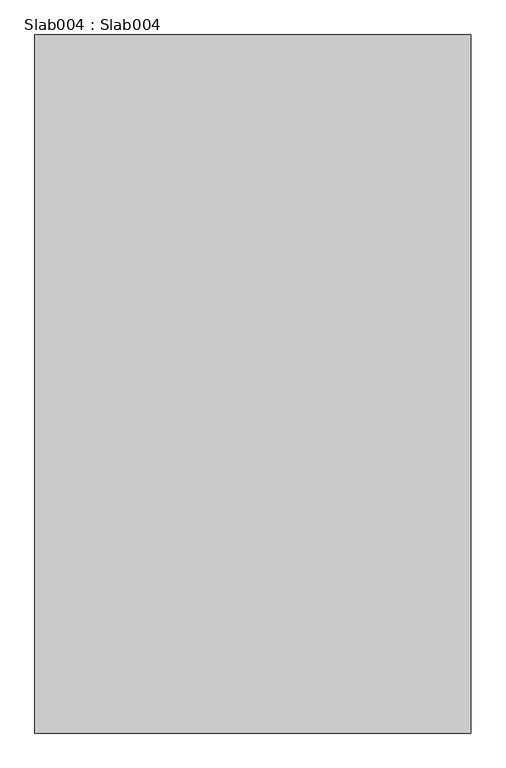
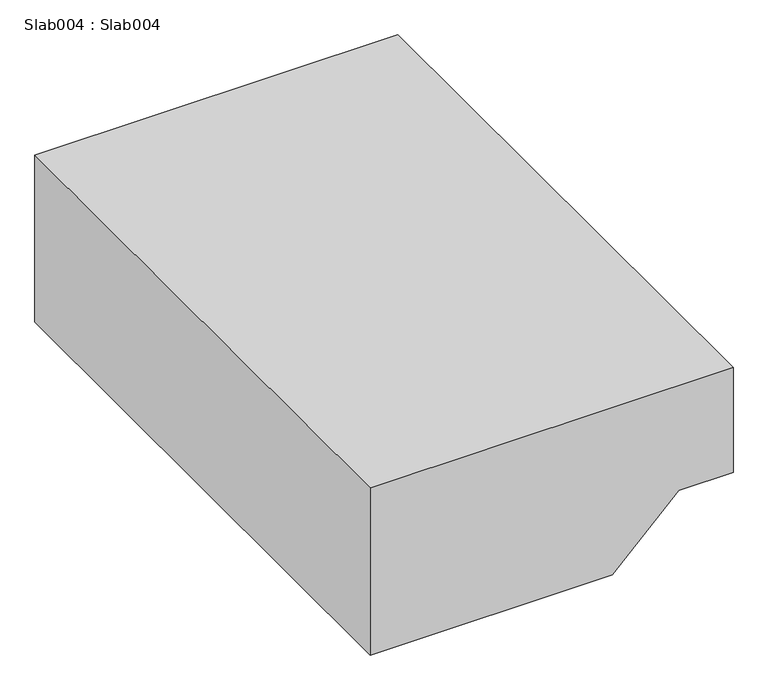
"""IFC4 building model written with IfcOpenShell, lengths in millimetres: proxy geometry, Slab004 : Slab004."""

from ifc_helpers import new_model, si_unit, frame, origin, place, context, project, spatial, polyline, outline, extrude, source, transform, mapped, element, save


def slab004_slab004_5b848ca3(model_context):
    return source(origin(), model_context, "Body", "SweptSolid", [
        extrude(outline(polyline([(32568.8960253, -10018.8790435), (31959.2960253, -10018.8790435), (31959.2960253, -9184.0737014), (32187.8960253, -8955.4737014), (32187.8960253, -8768.5299994), (32568.8960253, -8768.5299994), (32568.8960253, -10018.8790435)])), frame((0.0, 7982.1529359, 0.0), z_axis=(0.0, 1.0, 0.0), x_axis=(0.0, 0.0, 1.0)), (0.0, 0.0, 1.0), 2000.0),
    ])


if __name__ == "__main__":
    model = new_model("IFC4")
    model_context = context("Model", 3, world=origin())
    ifc_project = project(units=[si_unit("LENGTHUNIT", "METRE", prefix="MILLI")], contexts=[model_context])
    site = spatial("IfcSite", under=ifc_project)
    building = spatial("IfcBuilding", under=site)
    placement = place(None, origin())
    slab004_slab004_shape = slab004_slab004_5b848ca3(model_context)
    element("IfcBuildingElementProxy", 1, Name="Slab004 : Slab004", ObjectType="Slab004 : Slab004", at=placement, inside=building, context=model_context, shape_type="MappedRepresentation", body=[
        mapped(slab004_slab004_shape, transform((0.0, 0.0, 0.0), x_axis=(1.0, 0.0, 0.0), y_axis=(0.0, 1.0, 0.0), z_axis=(0.0, 0.0, 1.0))),
    ])
    save(model, "model.ifc")

# Revit data of these elements
# Type "Slab004 : Slab004"
#   NameOverride = "Slab004"
# Element 1 (IfcBuildingElementProxy, "Slab004 : Slab004")
#   Materials on its faces: "CONCRETE SLAB W/ GRADE BEAM (SEE STRUCT DWGS)"
# Materials
#   "CONCRETE SLAB W/ GRADE BEAM (SEE STRUCT DWGS)": class "Unassigned", colour RGB 128 128 128, transparency 0, Cost = 0
